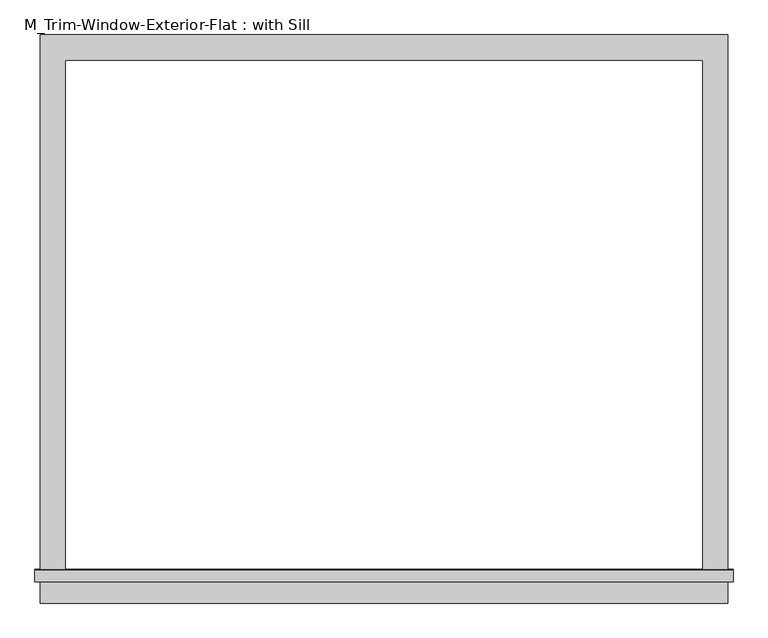
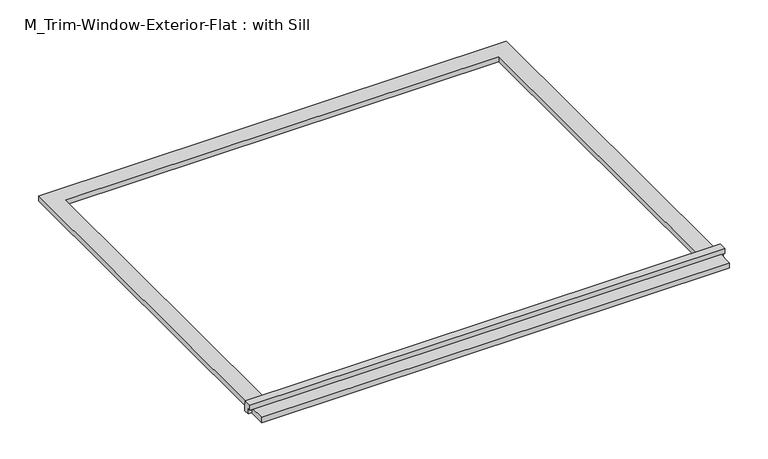
"""IFC4 building model written with IfcOpenShell, lengths in millimetres: proxy geometry, M_Trim-Window-Exterior-Flat : with Sill."""

from ifc_helpers import new_model, si_unit, frame, origin, origin_with_axes, place, context, project, spatial, polyline, outline, extrude, source, transform, mapped, element, save


def m_trim_window_exterior_flat_with_sill_e665999b(model_context):
    return source(origin(), model_context, "Body", "SweptSolid", [
        extrude(outline(polyline([(822.0, -1239.6323709), (822.0, -1299.6323709), (-822.0, -1299.6323709), (-822.0, -1239.6323709), (822.0, -1239.6323709)])), origin_with_axes(), (0.0, 0.0, 1.0), 19.05),
        extrude(outline(polyline([(-1249.2, 38.1), (-1221.6580645, 38.1), (-1219.2, 19.05), (-1219.2, 0.0), (-1239.6323709, 0.0), (-1239.6323709, 19.05), (-1249.2, 19.05), (-1249.2, 38.1)])), frame((-834.7, 0.0, 0.0), z_axis=(1.0, 0.0, 0.0), x_axis=(0.0, 1.0, 0.0)), (0.0, 0.0, 1.0), 1669.4),
        extrude(outline(polyline([(-822.0, 60.0), (822.0, 60.0), (822.0, -1219.2), (762.0, -1219.2), (762.0, 0.0), (-762.0, 0.0), (-762.0, -1219.2), (-822.0, -1219.2), (-822.0, 60.0)])), origin_with_axes(), (0.0, 0.0, 1.0), 19.05),
    ])


if __name__ == "__main__":
    model = new_model("IFC4")
    model_context = context("Model", 3, world=origin())
    ifc_project = project(units=[si_unit("LENGTHUNIT", "METRE", prefix="MILLI")], contexts=[model_context])
    site = spatial("IfcSite", under=ifc_project)
    building = spatial("IfcBuilding", under=site)
    placement = place(None, origin())
    m_trim_window_exterior_flat_with_sill_shape = m_trim_window_exterior_flat_with_sill_e665999b(model_context)
    element("IfcBuildingElementProxy", 1, Name="M_Trim-Window-Exterior-Flat : with Sill", ObjectType="M_Trim-Window-Exterior-Flat : with Sill", at=placement, inside=building, context=model_context, shape_type="MappedRepresentation", body=[
        mapped(m_trim_window_exterior_flat_with_sill_shape, transform((0.0, 0.0, 0.0), x_axis=(1.0, 0.0, 0.0), y_axis=(0.0, 1.0, 0.0), z_axis=(0.0, 0.0, 1.0))),
    ])
    save(model, "model.ifc")

# Revit data of these elements
# Type "M_Trim-Window-Exterior-Flat : with Sill"
#   Trim Width = 0' - 2.3622"
#   Trim Thickness_Picture Frame = 0' - 1.1811"
#   Trim Thickness_with Sill = 0' - 0 3/4"
#   Sill Thickness = 0' - 1.1811"
#   Opening Width [instance default] = 1' - 11.62205"
#   Opening Height [instance default] = 2' - 11.43307"
#   Default Elevation = 3' - 11.24409"
#   Sill = yes
#   Picture Frame = no
#   Trim Material [instance default] = none
# Element 1 (IfcBuildingElementProxy, "M_Trim-Window-Exterior-Flat : with Sill")
#   Opening Width = 5' - 0"
#   Opening Height = 4' - 0"
#   Trim Material = Clad - White
#   Materials on its faces: "Clad - White"
# Materials
#   "Clad - White": class "Wood", colour RGB 242 242 238, transparency 0, Cost = 0
